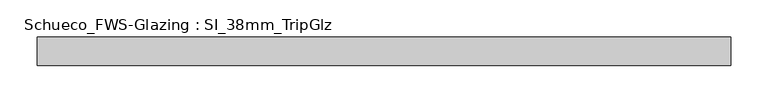
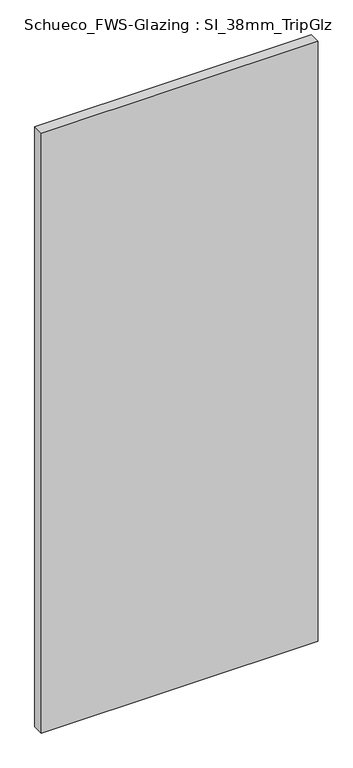
"""IFC4 building model written with IfcOpenShell, lengths in millimetres: plate geometry, Schueco_FWS-Glazing : SI_38mm_TripGlz."""

from ifc_helpers import new_model, si_unit, origin, origin_with_axes, place, context, project, spatial, polyline, outline, extrude, source, transform, mapped, element, save


def schueco_fws_glazing_si_38mm_tripglz_1b6edb7e(model_context):
    return source(origin(), model_context, "Body", "SweptSolid", [
        extrude(outline(polyline([(464.0, -38.0), (-464.0, -38.0), (-464.0, 0.0), (464.0, 0.0), (464.0, -38.0)])), origin_with_axes(), (0.0, 0.0, 1.0), 2128.0),
    ])


if __name__ == "__main__":
    model = new_model("IFC4")
    model_context = context("Model", 3, world=origin())
    ifc_project = project(units=[si_unit("LENGTHUNIT", "METRE", prefix="MILLI")], contexts=[model_context])
    site = spatial("IfcSite", under=ifc_project)
    building = spatial("IfcBuilding", under=site)
    placement = place(None, origin())
    schueco_fws_glazing_si_38mm_tripglz_shape = schueco_fws_glazing_si_38mm_tripglz_1b6edb7e(model_context)
    element("IfcPlate", 1, ObjectType="Schueco_FWS-Glazing : SI_38mm_TripGlz", at=placement, inside=building, context=model_context, shape_type="MappedRepresentation", body=[
        mapped(schueco_fws_glazing_si_38mm_tripglz_shape, transform((0.0, 0.0, 0.0), x_axis=(1.0, 0.0, 0.0), y_axis=(0.0, 1.0, 0.0), z_axis=(0.0, 0.0, 1.0))),
    ])
    save(model, "model.ifc")

# Revit data of these elements
# Type "Schueco_FWS-Glazing : SI_38mm_TripGlz"
#   Model = "Triple glazing 38mm"
#   Manufacturer = "Schueco International KG"
#   Analytic Construction = "<Keine Auswahl>"
#   Glazing thickness = 38 mm
#   FWS SI insert unit = yes
#   FWS HI insert unit = no
#   Glass = Glass
# Element 1 (IfcPlate, "Schueco_FWS-Glazing : SI_38mm_TripGlz")
#   Materials on its faces: "Glass"
# Materials
#   "Glass": class "Glass", colour RGB 128 128 255, transparency 0.75, Description = "Soda Lime Glass", Cost = 0
